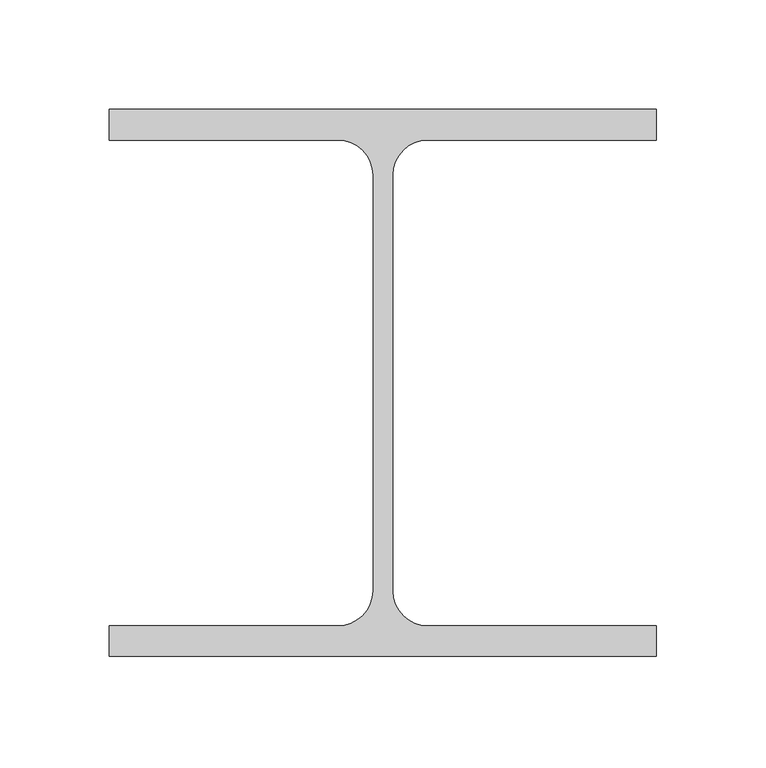
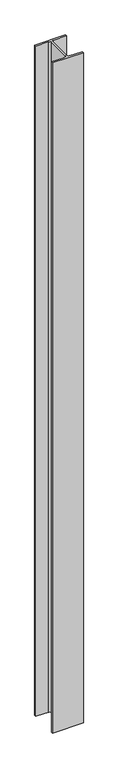
"""IFC4 building model written with IfcOpenShell, lengths in millimetres: column geometry, 0912_Steel Column_H_KSD3502 : H_SC_ASC_H-250x250x9x14."""

from ifc_helpers import new_model, si_unit, point, frame, frame_2d, origin, place, context, project, spatial, polyline, circle_curve, trimmed, segment, composite_curve, outline, extrude, source, transform, mapped, element, save


def column_c27b98d8(model_context):
    return source(origin(), model_context, "Body", "SweptSolid", [
        extrude(outline(composite_curve([segment(polyline([(125.0, 125.0), (125.0, 111.0), (20.5, 111.0)]), True, "CONTINUOUS"), segment(trimmed(circle_curve(frame_2d((20.5, 95.0)), 16.0), [point((20.5, 111.0))], [point((4.5, 95.0))], True, "CARTESIAN"), True, "CONTINUOUS"), segment(polyline([(4.5, 95.0), (4.5, -95.0)]), True, "CONTINUOUS"), segment(trimmed(circle_curve(frame_2d((20.5, -95.0)), 16.0), [point((4.5, -95.0))], [point((20.5, -111.0))], True, "CARTESIAN"), True, "CONTINUOUS"), segment(polyline([(20.5, -111.0), (125.0, -111.0), (125.0, -125.0), (-125.0, -125.0), (-125.0, -111.0), (-20.5, -111.0)]), True, "CONTINUOUS"), segment(trimmed(circle_curve(frame_2d((-20.5, -95.0)), 16.0), [point((-20.5, -111.0))], [point((-4.5, -95.0))], True, "CARTESIAN"), True, "CONTINUOUS"), segment(polyline([(-4.5, -95.0), (-4.5, 95.0)]), True, "CONTINUOUS"), segment(trimmed(circle_curve(frame_2d((-20.5, 95.0)), 16.0), [point((-4.5, 95.0))], [point((-20.5, 111.0))], True, "CARTESIAN"), True, "CONTINUOUS"), segment(polyline([(-20.5, 111.0), (-125.0, 111.0), (-125.0, 125.0), (125.0, 125.0)]), True, "CONTINUOUS")], self_intersect=False)), frame((0.0, 0.0, 599.9720055), z_axis=(0.0, 0.0, 1.0), x_axis=(1.0, 0.0, 0.0)), (0.0, 0.0, 1.0), 5750.0),
    ])


if __name__ == "__main__":
    model = new_model("IFC4")
    model_context = context("Model", 3, world=origin())
    ifc_project = project(units=[si_unit("LENGTHUNIT", "METRE", prefix="MILLI")], contexts=[model_context])
    site = spatial("IfcSite", under=ifc_project)
    building = spatial("IfcBuilding", under=site)
    placement = place(None, origin())
    column_shape = column_c27b98d8(model_context)
    element("IfcColumn", 1, ObjectType="0912_Steel Column_H_KSD3502 : H_SC_ASC_H-250x250x9x14", at=placement, inside=building, context=model_context, shape_type="MappedRepresentation", body=[
        mapped(column_shape, transform((0.0, 0.0, 0.0), x_axis=(1.0, 0.0, 0.0), y_axis=(0.0, 1.0, 0.0), z_axis=(0.0, 0.0, 1.0))),
    ])
    save(model, "model.ifc")

# Revit data of these elements
# Type "0912_Steel Column_H_KSD3502 : H_SC_ASC_H-250x250x9x14"
#   H_WM Code_1 = "S01AA002-00001 | Main Steel Structure Fabrication Work | Shelter/Building | Medium Steel - Standard (90KG/M>Weight≥30KG/M) | Material: (   )"
#   H_WM Code_2 = "S03AA028-00001 | Main Steel Structure Erection Work | Shelter/Building | Medium Steel (90KG/M>Weight≥30KG/M) | Material: (   )"
#   H_WM Code_3 = "S01AA010-00001 | Main Steel Structure Fabrication Work | Shelter/Building | Steel Painting/Coating | for Non-Fireproofed Steel Surface, Surface Preparation, Primer, Second & Final Coat | Material: (   )"
#   H_Q'ty Cal Type Tag = "SC-Q2"
#   Width = 25.0 cm
#   Web Thickness = 0.9 cm
#   Web Fillet = 1.6 cm
#   Warping Constant = 507646.0 cm⁶
#   Torsional Moment of Inertia = 51.4681 cm⁴
#   Section Area = 92.18 cm²
#   Plastic Modulus weak axis = 444.0 cm³
#   Plastic Modulus strong axis = 960.0 cm³
#   Perimeter = 1.46 m²/m
#   Nominal Weight = 72.40 kgf/m
#   Moment of Inertia weak axis = 3650.00 cm⁴
#   Moment of Inertia strong axis = 10800.00 cm⁴
#   Height = 25.0 cm
#   Flange Thickness = 1.4 cm
#   Elastic Modulus weak axis = 292.0 cm³
#   Elastic Modulus strong axis = 867.0 cm³
#   Centroid Vertical = 12.5 cm
#   Centroid Horizontal = 12.5 cm
#   Structural Material [instance default] = Steel, 45-345
#   Section Name Key = ""
#   Bolt Spacing = 0
#   Assembly Code = ""
# Element 1 (IfcColumn, "0912_Steel Column_H_KSD3502 : H_SC_ASC_H-250x250x9x14")
#   Structural Material = A03AD029-00005_Anchor Bolt (Installation only)_M24
#   Materials on its faces: "A03AD029-00005_Anchor Bolt (Installation only)_M24"
# Materials
#   "Steel, 45-345": class "Metal", colour RGB 189 187 185, transparency 0, Description = "Steel 345 MPa", Cost = 0
#   "A03AD029-00005_Anchor Bolt (Installation only)_M24": class "Unassigned", colour RGB 84 83 81, transparency 0, Cost = 0
